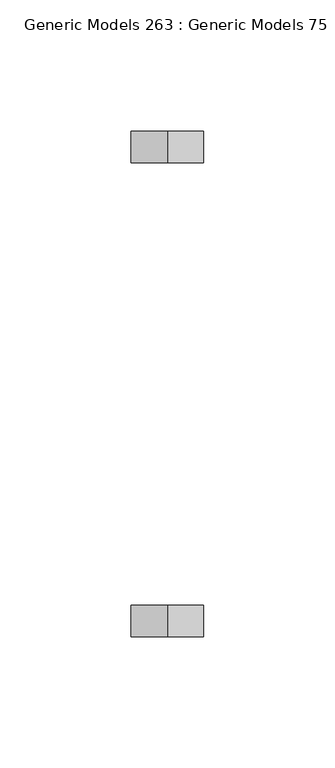
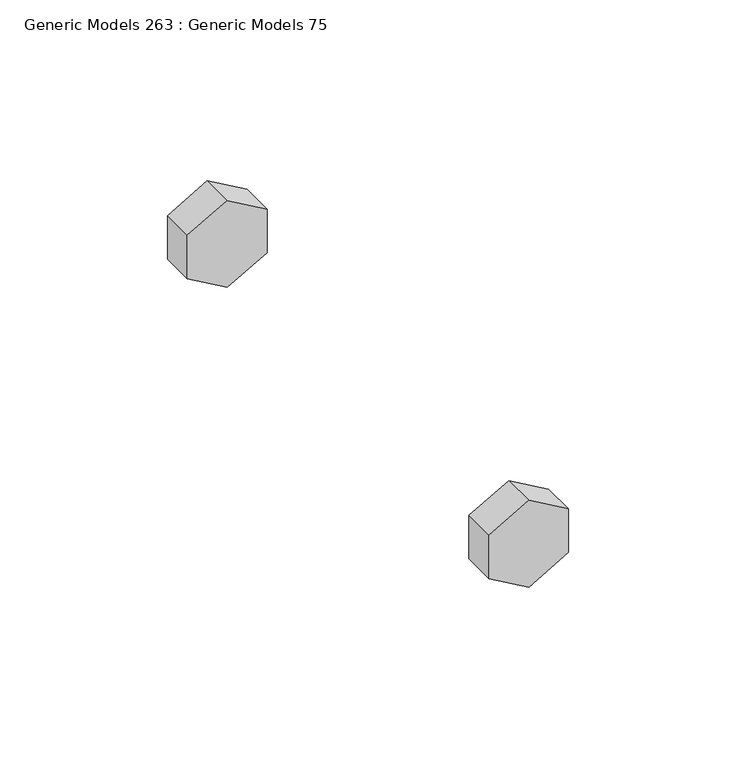
"""IFC4 building model written with IfcOpenShell, lengths in millimetres: proxy geometry, Generic Models 263 : Generic Models 75."""

from ifc_helpers import new_model, si_unit, frame, origin, place, context, project, spatial, polyline, outline, extrude, source, transform, mapped, element, save


def generic_models_263_generic_models_75_4b3c614c(model_context):
    return source(origin(), model_context, "Body", "SweptSolid", [
        extrude(outline(polyline([(268536.8902933, 31975.9942029), (268521.0537198, 31975.9942029), (268513.135433, 31989.7090778), (268521.0537198, 32003.4239528), (268536.8902933, 32003.4239528), (268544.80858, 31989.7090778), (268536.8902933, 31975.9942029)])), frame((0.0, 35373.9582942, 0.0), z_axis=(0.0, 1.0, 0.0), x_axis=(0.0, 0.0, 1.0)), (0.0, 0.0, 1.0), 11.90625),
        extrude(outline(polyline([(268536.8902933, 31975.9942029), (268521.0537198, 31975.9942029), (268513.135433, 31989.7090778), (268521.0537198, 32003.4239528), (268536.8902933, 32003.4239528), (268544.80858, 31989.7090778), (268536.8902933, 31975.9942029)])), frame((0.0, 35193.7770442, 0.0), z_axis=(0.0, 1.0, 0.0), x_axis=(0.0, 0.0, 1.0)), (0.0, 0.0, 1.0), 11.90625),
    ])


if __name__ == "__main__":
    model = new_model("IFC4")
    model_context = context("Model", 3, world=origin())
    ifc_project = project(units=[si_unit("LENGTHUNIT", "METRE", prefix="MILLI")], contexts=[model_context])
    site = spatial("IfcSite", under=ifc_project)
    building = spatial("IfcBuilding", under=site)
    placement = place(None, origin())
    generic_models_263_generic_models_75_shape = generic_models_263_generic_models_75_4b3c614c(model_context)
    element("IfcBuildingElementProxy", 1, Name="Generic Models 263 : Generic Models 75", ObjectType="Generic Models 263 : Generic Models 75", at=placement, inside=building, context=model_context, shape_type="MappedRepresentation", body=[
        mapped(generic_models_263_generic_models_75_shape, transform((0.0, 0.0, 0.0), x_axis=(1.0, 0.0, 0.0), y_axis=(0.0, 1.0, 0.0), z_axis=(0.0, 0.0, 1.0))),
    ])
    save(model, "model.ifc")

# Revit data of these elements
# Element 1 (IfcBuildingElementProxy, "Generic Models 263 : Generic Models 75")
#   Materials on its faces: "3/4\" GALV. THRU BOLTS"
# Materials
#   "3/4\" GALV. THRU BOLTS": class "Generic", colour RGB 105 69 171, transparency 0, Cost = 0
